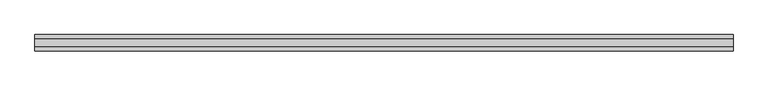
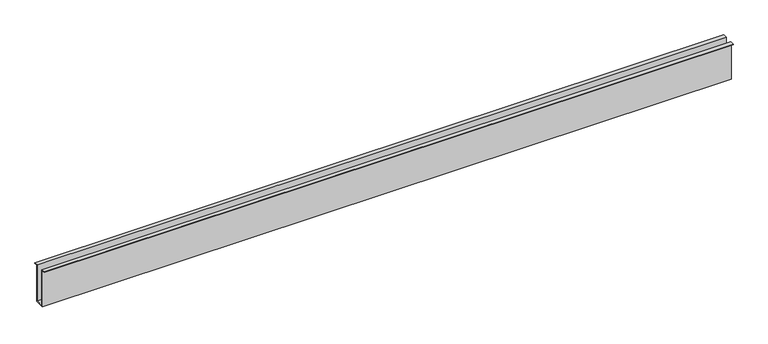
"""IFC4 building model written with IfcOpenShell, lengths in millimetres: railing geometry, ML_Perfil U de embutir3 : ML_Perfil U de embutir."""

from ifc_helpers import new_model, si_unit, frame, origin, place, context, project, spatial, polyline, outline, extrude, source, transform, mapped, element, save


def railing_81dbcb3b(model_context):
    return source(origin(), model_context, "Body", "SweptSolid", [
        extrude(outline(polyline([(1832.4523952, 3702.0), (1832.4523952, 3594.0), (1856.4523952, 3594.0), (1856.4523952, 3702.0), (1866.9523952, 3702.0), (1866.9523952, 3700.0), (1858.4523952, 3700.0), (1858.4523952, 3592.0), (1830.4523952, 3592.0), (1830.4523952, 3700.0), (1821.9523952, 3700.0), (1821.9523952, 3702.0), (1832.4523952, 3702.0)])), frame((-12226.1487231, 0.0, 0.0), z_axis=(1.0, 0.0, 0.0), x_axis=(0.0, 1.0, 0.0)), (0.0, 0.0, 1.0), 1940.0),
    ])


if __name__ == "__main__":
    model = new_model("IFC4")
    model_context = context("Model", 3, world=origin())
    ifc_project = project(units=[si_unit("LENGTHUNIT", "METRE", prefix="MILLI")], contexts=[model_context])
    site = spatial("IfcSite", under=ifc_project)
    building = spatial("IfcBuilding", under=site)
    placement = place(None, origin())
    railing_shape = railing_81dbcb3b(model_context)
    element("IfcRailing", 1, ObjectType="ML_Perfil U de embutir3 : ML_Perfil U de embutir", at=placement, inside=building, context=model_context, shape_type="MappedRepresentation", body=[
        mapped(railing_shape, transform((0.0, 0.0, 0.0), x_axis=(1.0, 0.0, 0.0), y_axis=(0.0, 1.0, 0.0), z_axis=(0.0, 0.0, 1.0))),
    ])
    save(model, "model.ifc")

# Revit data of these elements
# Type "ML_Perfil U de embutir3 : ML_Perfil U de embutir"
#   ME_Compr [instance default] = 1.94 m
#   ME_Material Perfil [instance default] = .ALUMÍNIO COM PINTURA ELETROSTÁTICA BRANCA
# Element 1 (IfcRailing, "ML_Perfil U de embutir3 : ML_Perfil U de embutir")
#   Materials on its faces: ".ALUMÍNIO COM PINTURA ELETROSTÁTICA BRANCA"
# Materials
#   ".ALUMÍNIO COM PINTURA ELETROSTÁTICA BRANCA": class "CC_METAIS", colour RGB 241 241 241, transparency 0, Cost = 0
